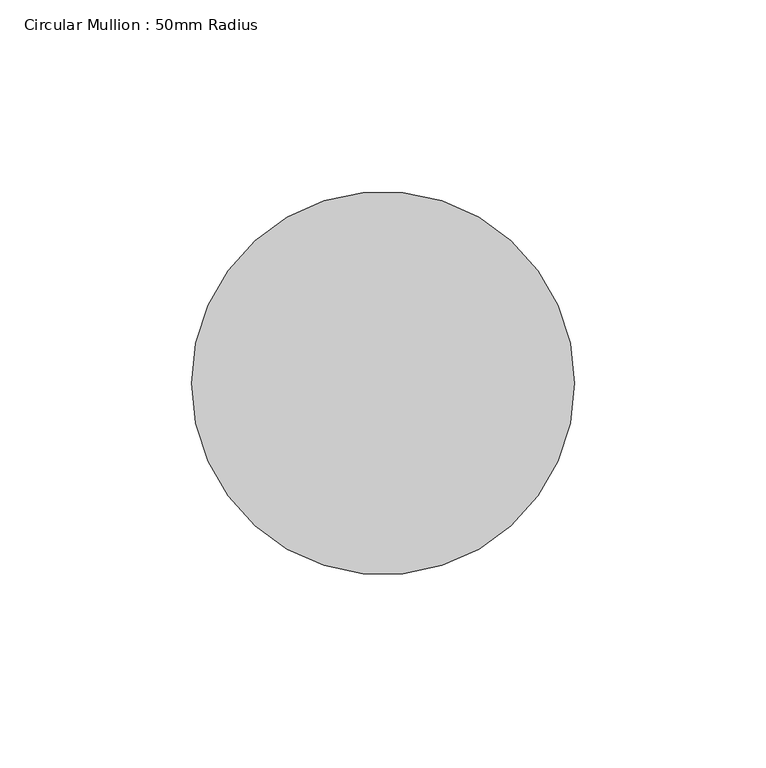
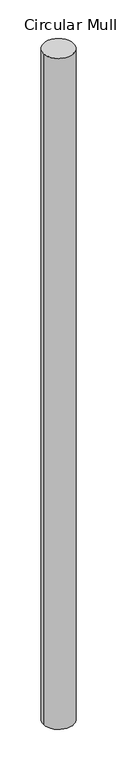
"""IFC4 building model written with IfcOpenShell, lengths in millimetres: member geometry, Circular Mullion : 50mm Radius."""

from ifc_helpers import new_model, si_unit, point, frame, origin, origin_2d, place, context, project, spatial, circle_curve, trimmed, segment, composite_curve, outline, extrude, source, transform, mapped, element, save


def circular_mullion_50mm_radius_2fcee45b(model_context):
    return source(origin(), model_context, "Body", "SweptSolid", [
        extrude(outline(composite_curve([segment(trimmed(circle_curve(origin_2d(), 50.0), [point((50.0, 0.0))], [point((-50.0, 0.0))], False, "CARTESIAN"), True, "CONTINUOUS"), segment(trimmed(circle_curve(origin_2d(), 50.0), [point((-50.0, 0.0))], [point((50.0, 0.0))], False, "CARTESIAN"), True, "CONTINUOUS")], self_intersect=False)), frame((0.0, 0.0, -2350.9847725), z_axis=(0.0, 0.0, 1.0), x_axis=(1.0, 0.0, 0.0)), (0.0, 0.0, 1.0), 2350.9847725),
    ])


if __name__ == "__main__":
    model = new_model("IFC4")
    model_context = context("Model", 3, world=origin())
    ifc_project = project(units=[si_unit("LENGTHUNIT", "METRE", prefix="MILLI")], contexts=[model_context])
    site = spatial("IfcSite", under=ifc_project)
    building = spatial("IfcBuilding", under=site)
    placement = place(None, origin())
    circular_mullion_50mm_radius_shape = circular_mullion_50mm_radius_2fcee45b(model_context)
    element("IfcMember", 1, ObjectType="Circular Mullion : 50mm Radius", at=placement, inside=building, context=model_context, shape_type="MappedRepresentation", body=[
        mapped(circular_mullion_50mm_radius_shape, transform((0.0, 0.0, 0.0), x_axis=(1.0, 0.0, 0.0), y_axis=(0.0, 1.0, 0.0), z_axis=(0.0, 0.0, 1.0))),
    ])
    save(model, "model.ifc")

# Revit data of these elements
# Type "Circular Mullion : 50mm Radius"
#   built-in parameter 1007350 = 0.164042 (stored number, unit not read)
# Element 1 (IfcMember, "Circular Mullion : 50mm Radius")
#   Materials on its faces: "Aluminium"
# Materials
#   "Aluminium": class "Metal", colour RGB 247 247 247, transparency 0, Description = "Aluminium 6061", Cost = 0
